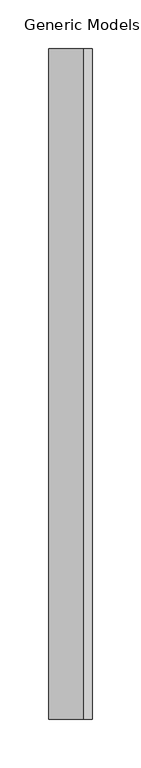
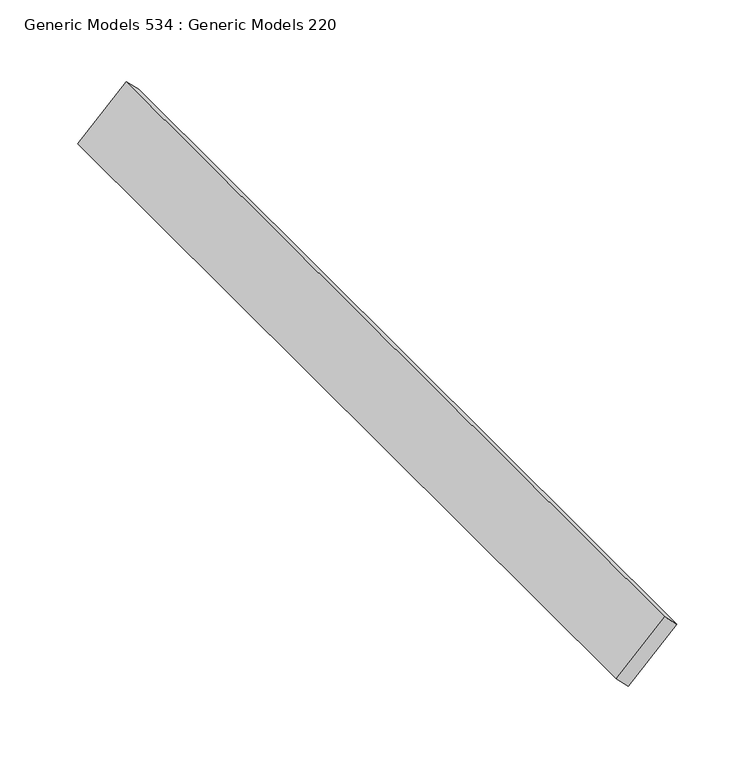
"""IFC4 building model written with IfcOpenShell, lengths in millimetres: proxy geometry, Generic Models 534 : Generic Models 220."""

from ifc_helpers import new_model, si_unit, frame, origin, place, context, project, spatial, polyline, outline, extrude, source, transform, mapped, element, save


def generic_models_534_generic_models_220_0aa05770(model_context):
    return source(origin(), model_context, "Body", "SweptSolid", [
        extrude(outline(polyline([(0.0, -12.7000001), (0.0, 0.0), (690.8142348, 0.0), (690.8142348, -12.7000001), (0.0, -12.7000001)])), frame((7841.3059863, 4539.4872686, 125192.1399101), z_axis=(0.7071067811868034, 0.0, 0.7071067811862918), x_axis=(0.0, -1.0, 0.0)), (0.0, 0.0, 1.0), 50.8),
    ])


if __name__ == "__main__":
    model = new_model("IFC4")
    model_context = context("Model", 3, world=origin())
    ifc_project = project(units=[si_unit("LENGTHUNIT", "METRE", prefix="MILLI")], contexts=[model_context])
    site = spatial("IfcSite", under=ifc_project)
    building = spatial("IfcBuilding", under=site)
    placement = place(None, origin())
    generic_models_534_generic_models_220_shape = generic_models_534_generic_models_220_0aa05770(model_context)
    element("IfcBuildingElementProxy", 1, Name="Generic Models 534 : Generic Models 220", ObjectType="Generic Models 534 : Generic Models 220", at=placement, inside=building, context=model_context, shape_type="MappedRepresentation", body=[
        mapped(generic_models_534_generic_models_220_shape, transform((0.0, 0.0, 0.0), x_axis=(1.0, 0.0, 0.0), y_axis=(0.0, 1.0, 0.0), z_axis=(0.0, 0.0, 1.0))),
    ])
    save(model, "model.ifc")

# Revit data of these elements
# Element 1 (IfcBuildingElementProxy, "Generic Models 534 : Generic Models 220")
#   Materials on its faces: "_WOOD TONE ALUMINUM EXTRUSION SLAT BY KNOTWOOD"
# Materials
#   "_WOOD TONE ALUMINUM EXTRUSION SLAT BY KNOTWOOD": class "Generic", colour RGB 177 130 114, transparency 0, Cost = 0
